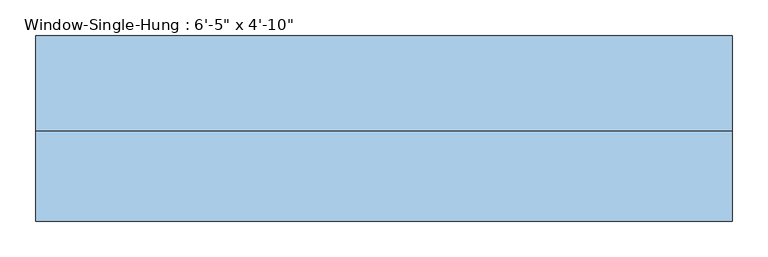
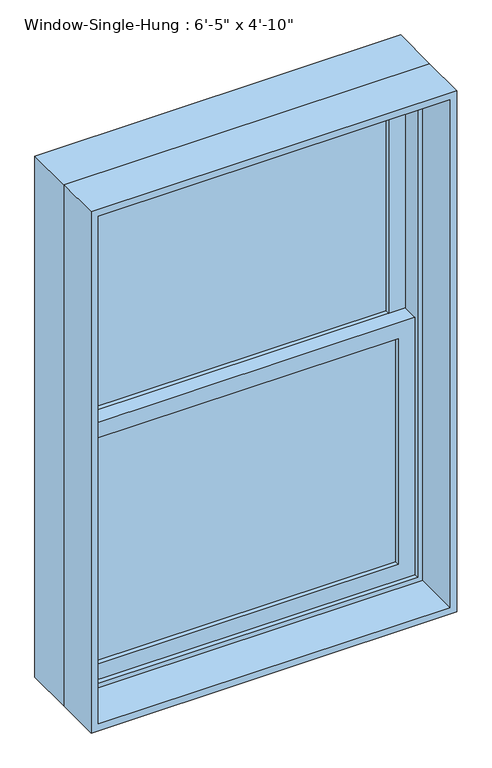
"""IFC4 building model written with IfcOpenShell, lengths in millimetres: window geometry."""

import ifcopenshell
import ifcopenshell.guid

model = None  # the IFC model being written
_history = None  # IfcOwnerHistory: only IFC2X3 demands one
_inside = {}  # id of a spatial element -> (the spatial element, [elements in it])
_under = {}  # id of a project, library or spatial element -> (it, [spatial elements below it])
_declared = {}  # id of a project -> (the project, [libraries it declares])
_typed = {}  # id of a type object -> (the type object, [elements of that type])
_made_of = {}  # id of a material, layer set ... -> (it, [elements and type objects made of it])


def new_model(schema):
    """Start an empty IFC model of exactly this schema.

    Asked for "IFC4X3", IfcOpenShell would pick the latest addendum, in which some entities
    have other attributes; the version numbers below select the first issue.
    IFC2X3 requires an IfcOwnerHistory on every rooted entity: one is made here for all.
    """
    global model, _history
    if schema == "IFC4X3":
        model = ifcopenshell.file(schema_version=(4, 3, 0, 0))
    else:
        model = ifcopenshell.file(schema=schema)
    _inside.clear()
    _under.clear()
    _declared.clear()
    _typed.clear()
    _made_of.clear()
    _history = None
    if model.schema == "IFC2X3":
        org = make("IfcOrganization", Name="unknown")
        user = make(
            "IfcPersonAndOrganization",
            ThePerson=make("IfcPerson", FamilyName="unknown"),
            TheOrganization=org,
        )
        app = make(
            "IfcApplication",
            ApplicationDeveloper=org,
            Version="unknown",
            ApplicationFullName="unknown",
            ApplicationIdentifier="unknown",
        )
        _history = make(
            "IfcOwnerHistory",
            OwningUser=user,
            OwningApplication=app,
            ChangeAction="ADDED",
            CreationDate=0,
        )
    return model


def make(cls, **values):
    """One entity of the class cls with the attributes given. An attribute that is None is left unset."""
    return model.create_entity(
        cls, **{name: value for name, value in values.items() if value is not None}
    )


def rooted(cls, **values):
    """An entity with a GlobalId (a new one), such as an element, a storey or a relation."""
    return make(cls, GlobalId=ifcopenshell.guid.new(), OwnerHistory=_history, **values)


def si_unit(unit_type, name, prefix=None):
    """IfcSIUnit, for example si_unit("LENGTHUNIT", "METRE", prefix="MILLI")."""
    return make("IfcSIUnit", UnitType=unit_type, Prefix=prefix, Name=name)


def assignment(units):
    """IfcUnitAssignment: the units of a project."""
    return None if units is None else make("IfcUnitAssignment", Units=units)


def point(xyz):
    """IfcCartesianPoint."""
    return None if xyz is None else make("IfcCartesianPoint", Coordinates=xyz)


def direction(xyz):
    """IfcDirection."""
    return None if xyz is None else make("IfcDirection", DirectionRatios=xyz)


def frame(location, z_axis=None, x_axis=None):
    """IfcAxis2Placement3D, a coordinate frame: its origin and axes. An axis left out is left unset."""
    return make(
        "IfcAxis2Placement3D",
        Location=point(location),
        Axis=direction(z_axis),
        RefDirection=direction(x_axis),
    )


def origin():
    """The frame at (0, 0, 0) with its axes left unset."""
    return frame((0.0, 0.0, 0.0))


def place(relative_to, where):
    """IfcLocalPlacement: puts the frame where relative to a parent placement (None: the world)."""
    return make(
        "IfcLocalPlacement", PlacementRelTo=relative_to, RelativePlacement=where
    )


def context(
    kind, dimensions, precision=None, world=None, true_north=None, identifier=None
):
    """IfcGeometricRepresentationContext, for example the 3D "Model" context."""
    return make(
        "IfcGeometricRepresentationContext",
        ContextIdentifier=identifier,
        ContextType=kind,
        CoordinateSpaceDimension=dimensions,
        Precision=precision,
        WorldCoordinateSystem=world,
        TrueNorth=true_north,
    )


def project(units=None, contexts=None):
    """IfcProject with its units and contexts."""
    return rooted(
        "IfcProject",
        Name="project",
        RepresentationContexts=contexts,
        UnitsInContext=assignment(units),
    )


def spatial(cls, under=None, at=None, **own):
    """A site, building, storey or space (cls), placed at a placement, below another one or the project."""
    s = rooted(cls, ObjectPlacement=at, **own)
    if under is not None:
        _under.setdefault(under.id(), (under, []))[1].append(s)
    return s


def polyline(points):
    """IfcPolyline through the points."""
    return make("IfcPolyline", Points=[point(p) for p in points])


def outline(outer, holes=None, kind="AREA"):
    """IfcArbitraryClosedProfileDef: a profile drawn as a closed curve; with holes, ...WithVoids."""
    if holes is None:
        return make("IfcArbitraryClosedProfileDef", ProfileType=kind, OuterCurve=outer)
    return make(
        "IfcArbitraryProfileDefWithVoids",
        ProfileType=kind,
        OuterCurve=outer,
        InnerCurves=holes,
    )


def extrude(swept, where, along, depth):
    """IfcExtrudedAreaSolid: the profile swept, set in the frame where, extruded along a direction by depth."""
    return make(
        "IfcExtrudedAreaSolid",
        SweptArea=swept,
        Position=where,
        ExtrudedDirection=direction(along),
        Depth=depth,
    )


def shape(context_of_items, identifier, shape_type, items):
    """IfcShapeRepresentation: the items that make up one representation, for example the "Body"."""
    return make(
        "IfcShapeRepresentation",
        ContextOfItems=context_of_items,
        RepresentationIdentifier=identifier,
        RepresentationType=shape_type,
        Items=items,
    )


def source(mapping_origin, context_of_items, identifier, shape_type, items):
    """IfcRepresentationMap: a shape defined once, which mapped items show again and again."""
    return make(
        "IfcRepresentationMap",
        MappingOrigin=mapping_origin,
        MappedRepresentation=shape(context_of_items, identifier, shape_type, items),
    )


def transform(
    local_origin,
    x_axis=None,
    y_axis=None,
    z_axis=None,
    scale=None,
    scale2=None,
    scale3=None,
    uniform=True,
):
    """IfcCartesianTransformationOperator3D, or its non-uniform kind. x_axis, y_axis, z_axis: its Axis1, 2, 3."""
    if uniform:
        return make(
            "IfcCartesianTransformationOperator3D",
            Axis1=direction(x_axis),
            Axis2=direction(y_axis),
            LocalOrigin=point(local_origin),
            Scale=scale,
            Axis3=direction(z_axis),
        )
    return make(
        "IfcCartesianTransformationOperator3DnonUniform",
        Axis1=direction(x_axis),
        Axis2=direction(y_axis),
        LocalOrigin=point(local_origin),
        Scale=scale,
        Axis3=direction(z_axis),
        Scale2=scale2,
        Scale3=scale3,
    )


def mapped(mapping_source, mapping_target):
    """IfcMappedItem: shows the shape of a source again, moved by a transform."""
    return make(
        "IfcMappedItem", MappingSource=mapping_source, MappingTarget=mapping_target
    )


def made_of(thing, what):
    """Note that an element or type object is made of a material, layer set ...; save() writes the relation."""
    if what is not None:
        _made_of.setdefault(what.id(), (what, []))[1].append(thing)
    return thing


def element(
    cls,
    number,
    at=None,
    inside=None,
    cuts=None,
    type_object=None,
    material=None,
    context=None,
    identifier="Body",
    shape_type=None,
    held_by="IfcProductDefinitionShape",
    body=None,
    shapes=None,
    **own,
):
    """One element of the class cls, such as IfcWall. Its Tag is "e" and its number.

    at: its placement. inside: the storey or other place that contains it. cuts: it is an
    opening in that element (IfcRelVoidsElement). A single representation is given by context,
    identifier, shape_type and body (its items); several are given by shapes. held_by: the class
    of the entity that holds the representations. save() writes the other relations.
    """
    e = rooted(cls, Tag="e%d" % number, ObjectPlacement=at, **own)
    if body is not None:
        shapes = [shape(context, identifier, shape_type, body)]
    if shapes is not None:
        e.Representation = make(held_by, Representations=shapes)
    if inside is not None:
        _inside.setdefault(inside.id(), (inside, []))[1].append(e)
    if cuts is not None:
        rooted(
            "IfcRelVoidsElement", RelatingBuildingElement=cuts, RelatedOpeningElement=e
        )
    if type_object is not None:
        _typed.setdefault(type_object.id(), (type_object, []))[1].append(e)
    return made_of(e, material)


def aggregate(whole, parts):
    """IfcRelAggregates: a whole, such as a stair, and the parts it consists of."""
    return rooted("IfcRelAggregates", RelatingObject=whole, RelatedObjects=parts)


def save(model, path):
    """Write the relations noted so far, then the file.

    IfcRelAggregates (storeys below a building ...), IfcRelContainedInSpatialStructure (elements
    in a storey), IfcRelDefinesByType, IfcRelAssociatesMaterial and IfcRelDeclares: one each for
    every whole, place, type object, material and project.
    """
    for whole, parts in _under.values():
        aggregate(whole, parts)
    for where, things in _inside.values():
        rooted(
            "IfcRelContainedInSpatialStructure",
            RelatedElements=things,
            RelatingStructure=where,
        )
    for kind, things in _typed.values():
        rooted("IfcRelDefinesByType", RelatedObjects=things, RelatingType=kind)
    for what, things in _made_of.values():
        rooted("IfcRelAssociatesMaterial", RelatedObjects=things, RelatingMaterial=what)
    for by, libraries in _declared.values():
        rooted("IfcRelDeclares", RelatingContext=by, RelatedDefinitions=libraries)
    model.write(path)


def window_979dede4(model_context):
    return source(origin(), model_context, "Body", "SweptSolid", [
        extrude(outline(polyline([(412.75, 50.8), (412.75, 44.45), (-412.75, 44.45), (-412.75, 50.8), (412.75, 50.8)])), frame((0.0, 0.0, 990.6), z_axis=(0.0, 0.0, 1.0), x_axis=(1.0, 0.0, 0.0)), (0.0, 0.0, 1.0), 638.175),
        extrude(outline(polyline([(-412.75, 38.1), (412.75, 38.1), (412.75, 31.75), (-412.75, 31.75), (-412.75, 38.1)])), frame((0.0, 0.0, 990.6), z_axis=(0.0, 0.0, 1.0), x_axis=(1.0, 0.0, 0.0)), (0.0, 0.0, 1.0), 638.175),
        extrude(outline(polyline([(412.75, 95.25), (412.75, 88.9), (-412.75, 88.9), (-412.75, 95.25), (412.75, 95.25)])), frame((0.0, 0.0, 1673.225), z_axis=(0.0, 0.0, 1.0), x_axis=(1.0, 0.0, 0.0)), (0.0, 0.0, 1.0), 638.175),
        extrude(outline(polyline([(-412.75, 82.55), (412.75, 82.55), (412.75, 76.2), (-412.75, 76.2), (-412.75, 82.55)])), frame((0.0, 0.0, 1673.225), z_axis=(0.0, 0.0, 1.0), x_axis=(1.0, 0.0, 0.0)), (0.0, 0.0, 1.0), 638.175),
        extrude(outline(polyline([(1673.225, -457.2), (946.15, -457.2), (946.15, 457.2), (1673.225, 457.2), (1673.225, -457.2)]), holes=[polyline([(1628.775, 412.75), (990.6, 412.75), (990.6, -412.75), (1628.775, -412.75), (1628.775, 412.75)])]), frame((0.0, 19.05, 0.0), z_axis=(0.0, 1.0, 0.0), x_axis=(0.0, 0.0, 1.0)), (0.0, 0.0, 1.0), 44.45),
        extrude(outline(polyline([(2355.85, -457.2), (1628.775, -457.2), (1628.775, 457.2), (2355.85, 457.2), (2355.85, -457.2)]), holes=[polyline([(2311.4, 412.75), (1673.225, 412.75), (1673.225, -412.75), (2311.4, -412.75), (2311.4, 412.75)])]), frame((0.0, 63.5, 0.0), z_axis=(0.0, 1.0, 0.0), x_axis=(0.0, 0.0, 1.0)), (0.0, 0.0, 1.0), 44.45),
        extrude(outline(polyline([(2387.6, -488.95), (914.4, -488.95), (914.4, 488.95), (2387.6, 488.95), (2387.6, -488.95)]), holes=[polyline([(2355.85, 457.2), (946.15, 457.2), (946.15, -457.2), (2355.85, -457.2), (2355.85, 457.2)])]), frame((0.0, 6.35, 0.0), z_axis=(0.0, 1.0, 0.0), x_axis=(0.0, 0.0, 1.0)), (0.0, 0.0, 1.0), 133.35),
        extrude(outline(polyline([(2387.6, 488.95), (2387.6, -488.95), (914.4, -488.95), (914.4, 488.95), (2387.6, 488.95)]), holes=[polyline([(2368.55, 469.9), (933.45, 469.9), (933.45, -469.9), (2368.55, -469.9), (2368.55, 469.9)])]), frame((0.0, -120.65, 0.0), z_axis=(0.0, 1.0, 0.0), x_axis=(0.0, 0.0, 1.0)), (0.0, 0.0, 1.0), 127.0),
    ])


if __name__ == "__main__":
    model = new_model("IFC4")
    model_context = context("Model", 3, world=origin())
    ifc_project = project(units=[si_unit("LENGTHUNIT", "METRE", prefix="MILLI")], contexts=[model_context])
    site = spatial("IfcSite", under=ifc_project)
    building = spatial("IfcBuilding", under=site)
    placement = place(None, origin())
    window_shape = window_979dede4(model_context)
    element("IfcWindow", 1, ObjectType="Window-Single-Hung : 6'-5\" x 4'-10\"", at=placement, inside=building, context=model_context, shape_type="MappedRepresentation", body=[
        mapped(window_shape, transform((0.0, 0.0, 0.0), x_axis=(1.0, 0.0, 0.0), y_axis=(0.0, 1.0, 0.0), z_axis=(0.0, 0.0, 1.0))),
    ])
    save(model, "model.ifc")

# Revit data of these elements
# Type "Window-Single-Hung : 6'-5\" x 4'-10\""
#   Type Mark = "01"
#   Fire Rating = "0.5h"
#   Construction Type Id = "DG-DR"
#   Assembly Code = "B2020100"
#   Analytic Construction = "Double glazing - domestic"
#   Wall Thickness [instance default] = 0' - 6"
#   Window Inset [instance default] = 0' - 0"
#   Visual Light Transmittance = 0.81
#   Thermal Resistance (R) = 0.319569 (m²·K)/W
#   Solar Heat Gain Coefficient = 0.76
#   Muntin Width = 2' - 8 1/2"
#   Muntin Height = 2' - 1 1/8"
#   Interior Wall Closure [instance default] = 0' - 1 1/2"
#   Rough Width = 3' - 3"
#   Rough Height = 4' - 10 1/2"
#   Frame Extension [instance default] = 0' - 1 1/4"
#   Exterior Wall Closure [instance default] = 0' - 0 1/2"
#   Extension Jamb [instance default] = 0' - 1 1/2"
#   Heat Transfer Coefficient (U) = 3.12929 W/(m²·K)
#   Height = 4' - 10"
#   Width = 3' - 2 1/2"
#   Top Muntin Visibility = no
#   Indicator Visibility = no
#   Extension Jamb Visibility [instance default] = yes
#   Interior Trim Visibility [instance default] = yes
#   Exterior Trim Visibility [instance default] = yes
#   Bottom Muntin Visibility = no
#   Muntin Pattern = Muntin Pattern_2x2 : Muntin Pattern_2x2
#   Interior Trim Material = 1X WOOD COMPOSITE TRIM
#   Interior Trim = Trim-Window-Interior-Flat : Picture Frame
#   Exterior Trim Material = 1X WOOD COMPOSITE TRIM
#   Exterior Trim = Trim-Window-Exterior-Flat : with Sill
#   Glass Panel Material = NEW DOUBLE HUNG WINDOWS (TYP.)
#   Exterior Frame Material = 1X WOOD COMPOSITE TRIM
#   Interior Frame Material = 1X WOOD COMPOSITE TRIM
#   Wall Closure = (empty or 0)
# Element 1 (IfcWindow, "Window-Single-Hung : 6'-5\" x 4'-10\"")
#   Wall Thickness = 0' - 9 1/2"
#   Extension Jamb = 0' - 5"
#   Materials on its faces: "1X WOOD COMPOSITE TRIM", "NEW DOUBLE HUNG WINDOWS (TYP.)"
# Materials
#   "1X WOOD COMPOSITE TRIM": class "Generic", colour RGB 88 61 61, transparency 0, Cost = 0
#   "NEW DOUBLE HUNG WINDOWS (TYP.)": class "Glass", colour RGB 218 227 224, transparency 0.85, Description = "Soda Lime Glass", Cost = 0
